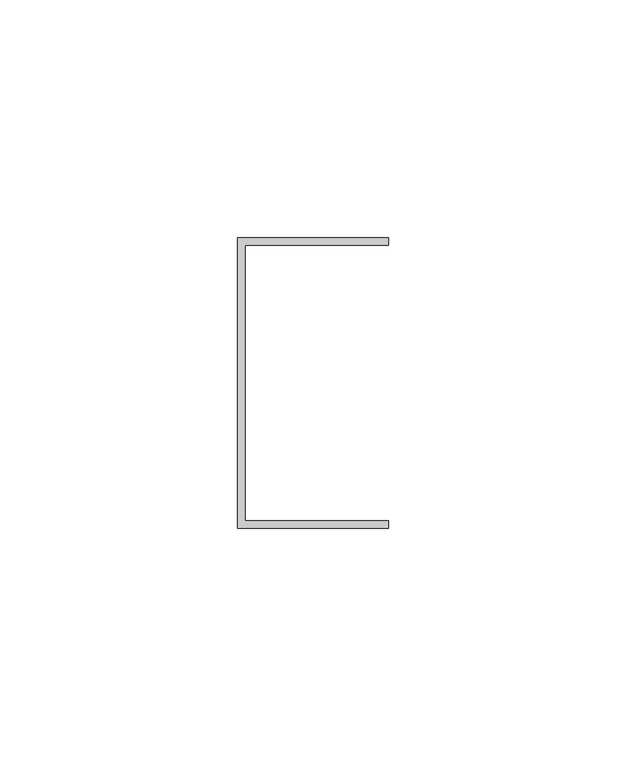
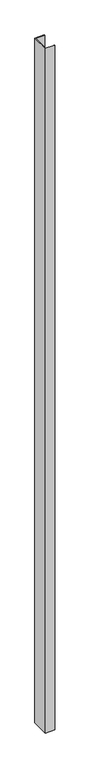
"""IFC4 building model written with IfcOpenShell, lengths in millimetres: proxy geometry, Generic Models 7:Generic Models 1:3:Generic Models 1:3 : Generic Models 7:Generic Models 1:305549:3:Generic Models 1:3:Generic Models 1:3 : Generic Models 7:Generic Models 1:305549:3 : Generic Models 7:Generic Models 1:3:Generic Models 1:3 : Generic Models 7:Generic Models 1:305549:301244:9 : Generic Models 7:Generic Models 1:3:Generic Models 1:3 : Generic Models 7:Generic Models 1:305549:3:Generic Models 1:3:Generic Models 1:3 : Generic Models 7:Generic Models 1:305549:3 : Generic Models 7:Generic Models 1:3:Generic Models 1:3 : Generic Models 7:Generic Models 1:305549:301244:308848."""

from ifc_helpers import new_model, si_unit, frame, origin, place, context, project, spatial, polyline, outline, extrude, source, transform, mapped, element, save


def generic_models_73bb5645(model_context):
    return source(origin(), model_context, "Body", "SweptSolid", [
        extrude(outline(polyline([(560352.9617238, -579015.772634), (560384.7117238, -579015.772634), (560384.7117238, -579017.360134), (560354.5492238, -579017.360134), (560354.5492238, -579075.303884), (560384.7117238, -579075.303884), (560384.7117238, -579076.891384), (560352.9617238, -579076.891384), (560352.9617238, -579015.772634)])), frame((0.0, 0.0, 3721.1), z_axis=(0.0, 0.0, 1.0), x_axis=(1.0, 0.0, 0.0)), (0.0, 0.0, 1.0), 2430.9324376),
    ])


if __name__ == "__main__":
    model = new_model("IFC4")
    model_context = context("Model", 3, world=origin())
    ifc_project = project(units=[si_unit("LENGTHUNIT", "METRE", prefix="MILLI")], contexts=[model_context])
    site = spatial("IfcSite", under=ifc_project)
    building = spatial("IfcBuilding", under=site)
    placement = place(None, origin())
    generic_models_shape = generic_models_73bb5645(model_context)
    element("IfcBuildingElementProxy", 1, Name="Generic Models 7:Generic Models 1:3:Generic Models 1:3 : Generic Models 7:Generic Models 1:305549:3:Generic Models 1:3:Generic Models 1:3 : Generic Models 7:Generic Models 1:305549:3 : Generic Models 7:Generic Models 1:3:Generic Models 1:3 : Generic Models 7:Generic Models 1:305549:301244:9 : Generic Models 7:Generic Models 1:3:Generic Models 1:3 : Generic Models 7:Generic Models 1:305549:3:Generic Models 1:3:Generic Models 1:3 : Generic Models 7:Generic Models 1:305549:3 : Generic Models 7:Generic Models 1:3:Generic Models 1:3 : Generic Models 7:Generic Models 1:305549:301244:308848", ObjectType="Generic Models 7:Generic Models 1:3:Generic Models 1:3 : Generic Models 7:Generic Models 1:305549:3:Generic Models 1:3:Generic Models 1:3 : Generic Models 7:Generic Models 1:305549:3 : Generic Models 7:Generic Models 1:3:Generic Models 1:3 : Generic Models 7:Generic Models 1:305549:301244:9 : Generic Models 7:Generic Models 1:3:Generic Models 1:3 : Generic Models 7:Generic Models 1:305549:3:Generic Models 1:3:Generic Models 1:3 : Generic Models 7:Generic Models 1:305549:3 : Generic Models 7:Generic Models 1:3:Generic Models 1:3 : Generic Models 7:Generic Models 1:305549:301244:308848", at=placement, inside=building, context=model_context, shape_type="MappedRepresentation", body=[
        mapped(generic_models_shape, transform((0.0, 0.0, 0.0), x_axis=(1.0, 0.0, 0.0), y_axis=(0.0, 1.0, 0.0), z_axis=(0.0, 0.0, 1.0))),
    ])
    save(model, "model.ifc")

# Revit data of these elements
# Type "Generic Models 7:Generic Models 1:3:Generic Models 1:3 : Generic Models 7:Generic Models 1:305549:3:Generic Models 1:3:Generic Models 1:3 : Generic Models 7:Generic Models 1:305549:3 : Generic Models 7:Generic Models 1:3:Generic Models 1:3 : Generic Models 7:Generic Models 1:305549:301244:9 : Generic Models 7:Generic Models 1:3:Generic Models 1:3 : Generic Models 7:Generic Models 1:305549:3:Generic Models 1:3:Generic Models 1:3 : Generic Models 7:Generic Models 1:305549:3 : Generic Models 7:Generic Models 1:3:Generic Models 1:3 : Generic Models 7:Generic Models 1:305549:301244:308848"
#   NameOverride = "Generic Models 7:Generic Models 1:3:Generic Models 1:3 : Generic Models 7:Generic Models 1:305549:3:Generic Models 1:3:Generic Models 1:3 : Generic Models 7:Generic Models 1:305549:3 : Generic Models 7:Generic Models 1:3:Generic Models 1:3 : Generic Models 7:Generic Models 1:305549:301244:308848"
#   ObjectTypeOverride = "Generic Models 1:3:Generic Models 1:3 : Generic Models 7:Generic Models 1:305549:3 : Generic Models 7:Generic Models 1:3:Generic Models 1:3 : Generic Models 7:Generic Models 1:305549:301244"
#   Reference = "Generic Models 1"
#   Tag = "308848"
# Element 1 (IfcBuildingElementProxy, "Generic Models 7:Generic Models 1:3:Generic Models 1:3 : Generic Models 7:Generic Models 1:305549:3:Generic Models 1:3:Generic Models 1:3 : Generic Models 7:Generic Models 1:305549:3 : Generic Models 7:Generic Models 1:3:Generic Models 1:3 : Generic Models 7:Generic Models 1:305549:301244:9 : Generic Models 7:Generic Models 1:3:Generic Models 1:3 : Generic Models 7:Generic Models 1:305549:3:Generic Models 1:3:Generic Models 1:3 : Generic Models 7:Generic Models 1:305549:3 : Generic Models 7:Generic Models 1:3:Generic Models 1:3 : Generic Models 7:Generic Models 1:305549:301244:308848")
#   Materials on its faces: "GALVANIZED U-CHANNEL (250T125-33)"
# Materials
#   "GALVANIZED U-CHANNEL (250T125-33)": class "Unassigned", colour RGB 202 201 200, transparency 0, Keynote = "M05451300.02", Cost = 0
